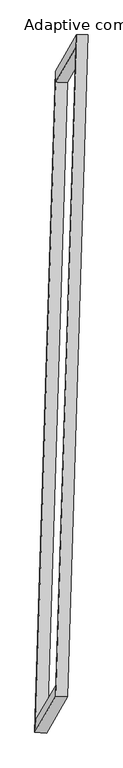
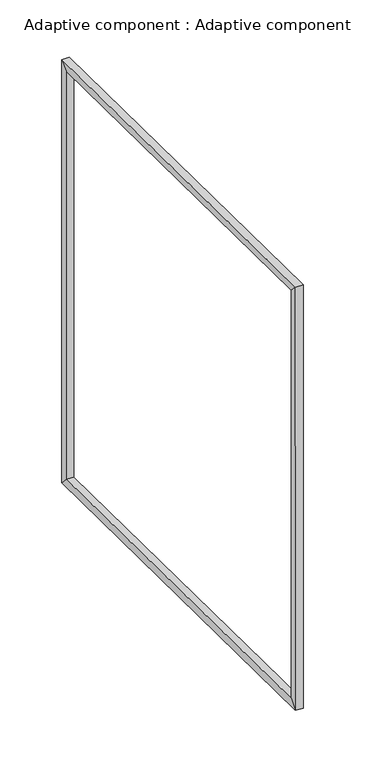
"""IFC4 building model written with IfcOpenShell, lengths in millimetres: proxy geometry, Adaptive component : Adaptive component."""

from ifc_helpers import new_model, si_unit, origin, place, context, project, spatial, faceted_brep, source, transform, mapped, element, save


def adaptive_component_adaptive_component_0a4da6c9(model_context):
    return source(origin(), model_context, "Body", "Brep", [
        faceted_brep([(91.9851339, 1490.522618, 3060.7621889), (157.0110727, 1490.3424918, 3060.5709272), (41.923315, 1292.9485098, -572.4525246), (-22.9853171, 1293.3298357, -568.5581944), (89.7615469, 1422.0955995, 2999.4485928), (-21.1005293, 1231.9493397, -500.1810012), (154.7874857, 1421.9154734, 2999.2573311), (43.8081028, 1231.5680138, -504.0753314), (-71.1892691, -2333.05119, -371.8569592), (-135.982389, -2328.9669394, -368.1674802), (-130.0520711, -2260.661682, -306.9646911), (-65.2589512, -2264.7459325, -310.6541701), (43.8984886, -2135.6572079, 3261.1664926), (-21.0119379, -2131.7741571, 3261.1529031), (-19.1899949, -2070.5154221, 3192.664903), (45.7204317, -2074.3984729, 3192.6784924)], [[[0, 1, 2, 3]], [[4, 0, 3, 5]], [[6, 4, 5, 7]], [[1, 6, 7, 2]], [[3, 2, 8, 9]], [[5, 3, 9, 10]], [[7, 5, 10, 11]], [[2, 7, 11, 8]], [[9, 8, 12, 13]], [[10, 9, 13, 14]], [[11, 10, 14, 15]], [[8, 11, 15, 12]], [[13, 12, 1, 0]], [[14, 13, 0, 4]], [[15, 14, 4, 6]], [[12, 15, 6, 1]]]),
    ])


if __name__ == "__main__":
    model = new_model("IFC4")
    model_context = context("Model", 3, world=origin())
    ifc_project = project(units=[si_unit("LENGTHUNIT", "METRE", prefix="MILLI")], contexts=[model_context])
    site = spatial("IfcSite", under=ifc_project)
    building = spatial("IfcBuilding", under=site)
    placement = place(None, origin())
    adaptive_component_adaptive_component_shape = adaptive_component_adaptive_component_0a4da6c9(model_context)
    element("IfcBuildingElementProxy", 1, Name="Adaptive component : Adaptive component", ObjectType="Adaptive component : Adaptive component", at=placement, inside=building, context=model_context, shape_type="MappedRepresentation", body=[
        mapped(adaptive_component_adaptive_component_shape, transform((0.0, 0.0, 0.0), x_axis=(1.0, 0.0, 0.0), y_axis=(0.0, 1.0, 0.0), z_axis=(0.0, 0.0, 1.0))),
    ])
    save(model, "model.ifc")

# Revit data of these elements
# Type "Adaptive component : Adaptive component"
#   r [instance default] = 2063.125 mm
#   2r [instance default] = 4126.251 mm
#   Number [instance default] = 5
#   Default Elevation = 0
# Element 1 (IfcBuildingElementProxy, "Adaptive component : Adaptive component")
#   r = 2477.313 mm
#   2r = 4954.626 mm
#   Number = 20
